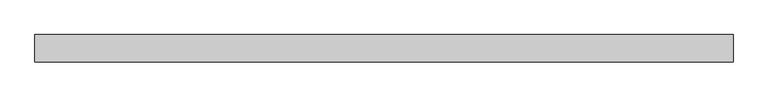
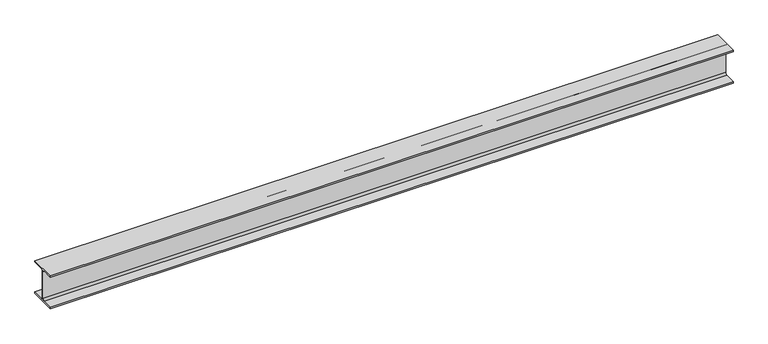
"""IFC4 building model written with IfcOpenShell, lengths in millimetres: beam geometry, 0912_Steel Framing_H-KSD3502 : H_SB_ASB_H-390x300x10x16."""

from ifc_helpers import new_model, si_unit, point, frame, frame_2d, origin, place, context, project, spatial, polyline, circle_curve, trimmed, segment, composite_curve, outline, extrude, source, transform, mapped, element, save


def beam_3fa8158e(model_context):
    return source(origin(), model_context, "Body", "SweptSolid", [
        extrude(outline(composite_curve([segment(polyline([(150.0, -179.0), (150.0, -195.0), (-150.0, -195.0), (-150.0, -179.0), (-27.0, -179.0)]), True, "CONTINUOUS"), segment(trimmed(circle_curve(frame_2d((-27.0, -157.0)), 22.0), [point((-27.0, -179.0))], [point((-5.0, -157.0))], True, "CARTESIAN"), True, "CONTINUOUS"), segment(polyline([(-5.0, -157.0), (-5.0, 157.0)]), True, "CONTINUOUS"), segment(trimmed(circle_curve(frame_2d((-27.0, 157.0)), 22.0), [point((-5.0, 157.0))], [point((-27.0, 179.0))], True, "CARTESIAN"), True, "CONTINUOUS"), segment(polyline([(-27.0, 179.0), (-150.0, 179.0), (-150.0, 195.0), (150.0, 195.0), (150.0, 179.0), (27.0, 179.0)]), True, "CONTINUOUS"), segment(trimmed(circle_curve(frame_2d((27.0, 157.0)), 22.0), [point((27.0, 179.0))], [point((5.0, 157.0))], True, "CARTESIAN"), True, "CONTINUOUS"), segment(polyline([(5.0, 157.0), (5.0, -157.0)]), True, "CONTINUOUS"), segment(trimmed(circle_curve(frame_2d((27.0, -157.0)), 22.0), [point((5.0, -157.0))], [point((27.0, -179.0))], True, "CARTESIAN"), True, "CONTINUOUS"), segment(polyline([(27.0, -179.0), (150.0, -179.0)]), True, "CONTINUOUS")], self_intersect=False)), frame((-3837.3, 0.0, 0.0), z_axis=(1.0, 0.0, 0.0), x_axis=(0.0, 1.0, 0.0)), (0.0, 0.0, 1.0), 7674.6),
    ])


if __name__ == "__main__":
    model = new_model("IFC4")
    model_context = context("Model", 3, world=origin())
    ifc_project = project(units=[si_unit("LENGTHUNIT", "METRE", prefix="MILLI")], contexts=[model_context])
    site = spatial("IfcSite", under=ifc_project)
    building = spatial("IfcBuilding", under=site)
    placement = place(None, origin())
    beam_shape = beam_3fa8158e(model_context)
    element("IfcBeam", 1, ObjectType="0912_Steel Framing_H-KSD3502 : H_SB_ASB_H-390x300x10x16", at=placement, inside=building, context=model_context, shape_type="MappedRepresentation", body=[
        mapped(beam_shape, transform((0.0, 0.0, 0.0), x_axis=(1.0, 0.0, 0.0), y_axis=(0.0, 1.0, 0.0), z_axis=(0.0, 0.0, 1.0))),
    ])
    save(model, "model.ifc")

# Revit data of these elements
# Type "0912_Steel Framing_H-KSD3502 : H_SB_ASB_H-390x300x10x16"
#   H_WM Code_1 = "S01AA001-00001 | Main Steel Structure Fabrication Work | Shelter/Building | Heavy Steel - Standard (Weight≥90KG/M) | Material: (   )"
#   H_WM Code_2 = "S03AA027-00001 | Main Steel Structure Erection Work | Shelter/Building | Heavy Steel (Weight≥90KG/M) | Material: (   )"
#   H_WM Code_3 = "S01AA010-00001 | Main Steel Structure Fabrication Work | Shelter/Building | Steel Painting/Coating | for Non-Fireproofed Steel Surface, Surface Preparation, Primer, Second & Final Coat | Material: (   )"
#   H_Q'ty Cal Type Tag = "SB-Q2"
#   Width = 30.0 cm
#   Web Thickness = 1.0 cm
#   Web Fillet = 2.2 cm
#   Warping Constant = 2520000.0 cm⁶
#   W = 0
#   Torsional Moment of Inertia = 94.3867 cm⁴
#   Section Area = 136.0 cm²
#   Plastic Modulus weak axis = 733.0 cm³
#   Plastic Modulus strong axis = 2190.0 cm³
#   Perimeter = 1.92 m²/m
#   Nominal Weight = 107.00 kgf/m
#   Moment of Inertia weak axis = 7210.00 cm⁴
#   Moment of Inertia strong axis = 38700.00 cm⁴
#   Height = 39.0 cm
#   Flange Thickness = 1.6 cm
#   Elastic Modulus weak axis = 481.0 cm³
#   Elastic Modulus strong axis = 1980.0 cm³
#   Centroid Vertical = 19.5 cm
#   Centroid Horizontal = 15.0 cm
#   Ix = 387000000
#   Length [instance default] = 1.5240 m
#   Zx = 2190000
#   b = 0.3000 m
#   h = 0.3900 m
#   r = 0.0220 m
#   s = 0.0100 m
#   t = 0.0160 m
#   A = 0.0136 m²
#   Structural Material [instance default] = Steel, 45-345
#   Assembly Code = ""
# Element 1 (IfcBeam, "0912_Steel Framing_H-KSD3502 : H_SB_ASB_H-390x300x10x16")
#   Structural Material = none
# Materials
#   "Steel, 45-345": class "Metal", colour RGB 189 187 185, transparency 0, Description = "Steel 345 MPa", Cost = 0
